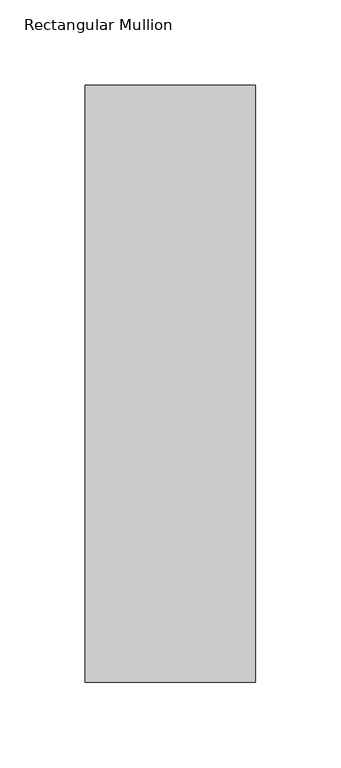
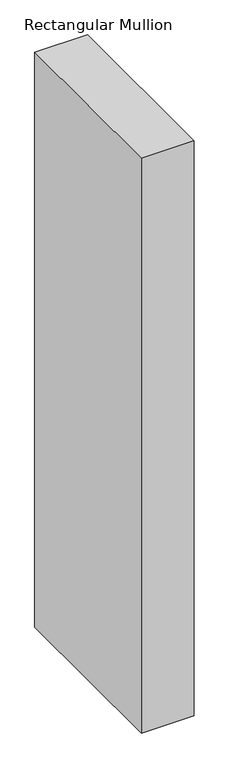
"""IFC4 building model written with IfcOpenShell, lengths in millimetres: member geometry, Rectangular Mullion : WWm-100x350-100mmOffset."""

from ifc_helpers import new_model, si_unit, frame, origin, place, context, project, spatial, polyline, outline, extrude, source, transform, mapped, element, save


def rectangular_mullion_55d0ee2a(model_context):
    return source(origin(), model_context, "Body", "SweptSolid", [
        extrude(outline(polyline([(0.0, 175.0), (0.0, -175.0), (-100.0, -175.0), (-100.0, 175.0), (0.0, 175.0)])), frame((0.0, 0.0, -1150.0), z_axis=(0.0, 0.0, 1.0), x_axis=(1.0, 0.0, 0.0)), (0.0, 0.0, 1.0), 1150.0),
    ])


if __name__ == "__main__":
    model = new_model("IFC4")
    model_context = context("Model", 3, world=origin())
    ifc_project = project(units=[si_unit("LENGTHUNIT", "METRE", prefix="MILLI")], contexts=[model_context])
    site = spatial("IfcSite", under=ifc_project)
    building = spatial("IfcBuilding", under=site)
    placement = place(None, origin())
    rectangular_mullion_shape = rectangular_mullion_55d0ee2a(model_context)
    element("IfcMember", 1, ObjectType="Rectangular Mullion : WWm-100x350-100mmOffset", at=placement, inside=building, context=model_context, shape_type="MappedRepresentation", body=[
        mapped(rectangular_mullion_shape, transform((0.0, 0.0, 0.0), x_axis=(1.0, 0.0, 0.0), y_axis=(0.0, 1.0, 0.0), z_axis=(0.0, 0.0, 1.0))),
    ])
    save(model, "model.ifc")

# Revit data of these elements
# Type "Rectangular Mullion : WWm-100x350-100mmOffset"
#   built-in parameter 1007304 = 1.14829 (stored number, unit not read)
#   built-in parameter 1007301 = 0.164042 (stored number, unit not read)
#   built-in parameter 1007300 = 0.164042 (stored number, unit not read)
# Element 1 (IfcMember, "Rectangular Mullion : WWm-100x350-100mmOffset")
#   Materials on its faces: "WW-EC-RGB-Mullion"
# Materials
#   "WW-EC-RGB-Mullion": class "Generic", colour RGB 255 255 255, transparency 0, Comments = "If region requests black mullions, switch asset color to RGB 25-25-25", Description = "Generic Color", Cost = 0
